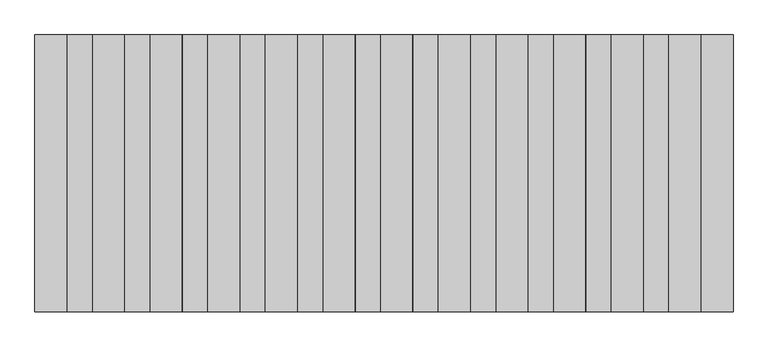
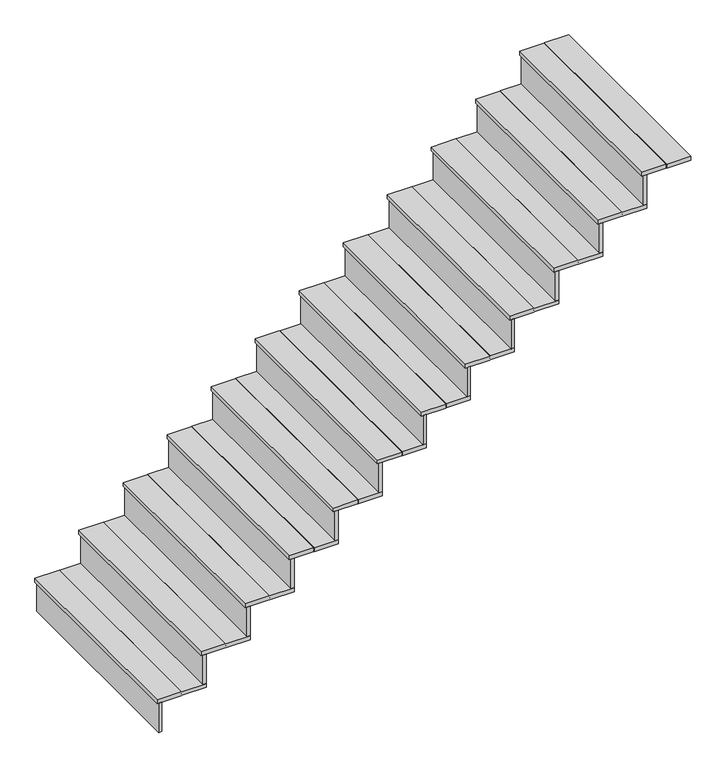
"""IFC4 building model written with IfcOpenShell, lengths in millimetres: stair flight geometry."""

from ifc_helpers import new_model, si_unit, frame, origin, place, context, project, spatial, polyline, outline, extrude, source, transform, mapped, element, save


def stair_flight_ee30e5b9(model_context):
    return source(origin(), model_context, "Body", "SweptSolid", [
        extrude(outline(polyline([(7016.9566393, -79669.5176951), (6997.9066393, -79669.5176951), (6997.9066393, -78450.3176951), (7016.9566393, -78450.3176951), (7016.9566393, -79669.5176951)])), frame((0.0, 0.0, -2438.4), z_axis=(0.0, 0.0, 1.0), x_axis=(1.0, 0.0, 0.0)), (0.0, 0.0, 1.0), 179.2882813),
        extrude(outline(polyline([(-2259.1117187, 7128.0816393), (-2247.3574467, 7128.0816393), (-2247.3574467, 7131.2566393), (-2259.1117188, 7131.2566393), (-2259.1117188, 7270.9566393), (-2235.2, 7270.9566393), (-2235.2, 7131.2566393), (-2246.9542721, 7131.2566393), (-2246.9542721, 7128.0816393), (-2235.2, 7128.0816393), (-2235.2, 6988.3816393), (-2259.1117187, 6988.3816393), (-2259.1117187, 7128.0816393)])), frame((0.0, -79669.5176951, 0.0), z_axis=(0.0, 1.0, 0.0), x_axis=(0.0, 0.0, 1.0)), (0.0, 0.0, 1.0), 1219.2),
        extrude(outline(polyline([(7270.9566393, -79669.5176951), (7251.9066393, -79669.5176951), (7251.9066393, -78450.3176951), (7270.9566393, -78450.3176951), (7270.9566393, -79669.5176951)])), frame((0.0, 0.0, -2235.2), z_axis=(0.0, 0.0, 1.0), x_axis=(1.0, 0.0, 0.0)), (0.0, 0.0, 1.0), 179.2882813),
        extrude(outline(polyline([(-2055.9117188, 7382.0816393), (-2044.1574467, 7382.0816393), (-2044.1574467, 7385.2566393), (-2055.9117188, 7385.2566393), (-2055.9117188, 7524.9566393), (-2032.0, 7524.9566393), (-2032.0, 7385.2566393), (-2043.7542721, 7385.2566393), (-2043.7542721, 7382.0816393), (-2032.0, 7382.0816393), (-2032.0, 7242.3816393), (-2055.9117188, 7242.3816393), (-2055.9117188, 7382.0816393)])), frame((0.0, -79669.5176951, 0.0), z_axis=(0.0, 1.0, 0.0), x_axis=(0.0, 0.0, 1.0)), (0.0, 0.0, 1.0), 1219.2),
        extrude(outline(polyline([(7524.9566393, -79669.5176951), (7505.9066393, -79669.5176951), (7505.9066393, -78450.3176951), (7524.9566393, -78450.3176951), (7524.9566393, -79669.5176951)])), frame((0.0, 0.0, -2032.0), z_axis=(0.0, 0.0, 1.0), x_axis=(1.0, 0.0, 0.0)), (0.0, 0.0, 1.0), 179.2882813),
        extrude(outline(polyline([(-1852.7117188, 7636.0816393), (-1840.9574467, 7636.0816393), (-1840.9574467, 7639.2566393), (-1852.7117188, 7639.2566393), (-1852.7117188, 7778.9566393), (-1828.8, 7778.9566393), (-1828.8, 7639.2566393), (-1840.5542721, 7639.2566393), (-1840.5542721, 7636.0816393), (-1828.8, 7636.0816393), (-1828.8, 7496.3816393), (-1852.7117188, 7496.3816393), (-1852.7117188, 7636.0816393)])), frame((0.0, -79669.5176951, 0.0), z_axis=(0.0, 1.0, 0.0), x_axis=(0.0, 0.0, 1.0)), (0.0, 0.0, 1.0), 1219.2),
        extrude(outline(polyline([(7778.9566393, -79669.5176951), (7759.9066393, -79669.5176951), (7759.9066393, -78450.3176951), (7778.9566393, -78450.3176951), (7778.9566393, -79669.5176951)])), frame((0.0, 0.0, -1828.8), z_axis=(0.0, 0.0, 1.0), x_axis=(1.0, 0.0, 0.0)), (0.0, 0.0, 1.0), 179.2882813),
        extrude(outline(polyline([(-1649.5117188, 7890.0816393), (-1637.7574467, 7890.0816393), (-1637.7574467, 7893.2566393), (-1649.5117188, 7893.2566393), (-1649.5117188, 8032.9566393), (-1625.6, 8032.9566393), (-1625.6, 7893.2566393), (-1637.3542721, 7893.2566393), (-1637.3542721, 7890.0816393), (-1625.6, 7890.0816393), (-1625.6, 7750.3816393), (-1649.5117188, 7750.3816393), (-1649.5117188, 7890.0816393)])), frame((0.0, -79669.5176951, 0.0), z_axis=(0.0, 1.0, 0.0), x_axis=(0.0, 0.0, 1.0)), (0.0, 0.0, 1.0), 1219.2),
        extrude(outline(polyline([(8032.9566393, -79669.5176951), (8013.9066393, -79669.5176951), (8013.9066393, -78450.3176951), (8032.9566393, -78450.3176951), (8032.9566393, -79669.5176951)])), frame((0.0, 0.0, -1625.6), z_axis=(0.0, 0.0, 1.0), x_axis=(1.0, 0.0, 0.0)), (0.0, 0.0, 1.0), 179.2882813),
        extrude(outline(polyline([(-1446.3117187, 8144.0816393), (-1434.5574467, 8144.0816393), (-1434.5574467, 8147.2566393), (-1446.3117188, 8147.2566393), (-1446.3117188, 8286.9566393), (-1422.4, 8286.9566393), (-1422.4, 8147.2566393), (-1434.1542721, 8147.2566393), (-1434.1542721, 8144.0816393), (-1422.4, 8144.0816393), (-1422.4, 8004.3816393), (-1446.3117187, 8004.3816393), (-1446.3117187, 8144.0816393)])), frame((0.0, -79669.5176951, 0.0), z_axis=(0.0, 1.0, 0.0), x_axis=(0.0, 0.0, 1.0)), (0.0, 0.0, 1.0), 1219.2),
        extrude(outline(polyline([(8286.9566393, -79669.5176951), (8267.9066393, -79669.5176951), (8267.9066393, -78450.3176951), (8286.9566393, -78450.3176951), (8286.9566393, -79669.5176951)])), frame((0.0, 0.0, -1422.4), z_axis=(0.0, 0.0, 1.0), x_axis=(1.0, 0.0, 0.0)), (0.0, 0.0, 1.0), 179.2882813),
        extrude(outline(polyline([(-1243.1117187, 8398.0816393), (-1231.3574467, 8398.0816393), (-1231.3574467, 8401.2566393), (-1243.1117188, 8401.2566393), (-1243.1117188, 8540.9566393), (-1219.2, 8540.9566393), (-1219.2, 8401.2566393), (-1230.9542721, 8401.2566393), (-1230.9542721, 8398.0816393), (-1219.2, 8398.0816393), (-1219.2, 8258.3816393), (-1243.1117187, 8258.3816393), (-1243.1117187, 8398.0816393)])), frame((0.0, -79669.5176951, 0.0), z_axis=(0.0, 1.0, 0.0), x_axis=(0.0, 0.0, 1.0)), (0.0, 0.0, 1.0), 1219.2),
        extrude(outline(polyline([(8540.9566393, -79669.5176951), (8521.9066393, -79669.5176951), (8521.9066393, -78450.3176951), (8540.9566393, -78450.3176951), (8540.9566393, -79669.5176951)])), frame((0.0, 0.0, -1219.2), z_axis=(0.0, 0.0, 1.0), x_axis=(1.0, 0.0, 0.0)), (0.0, 0.0, 1.0), 179.2882813),
        extrude(outline(polyline([(-1039.9117188, 8652.0816393), (-1028.1574467, 8652.0816393), (-1028.1574467, 8655.2566393), (-1039.9117188, 8655.2566393), (-1039.9117188, 8794.9566393), (-1016.0, 8794.9566393), (-1016.0, 8655.2566393), (-1027.7542721, 8655.2566393), (-1027.7542721, 8652.0816393), (-1016.0, 8652.0816393), (-1016.0, 8512.3816393), (-1039.9117188, 8512.3816393), (-1039.9117188, 8652.0816393)])), frame((0.0, -79669.5176951, 0.0), z_axis=(0.0, 1.0, 0.0), x_axis=(0.0, 0.0, 1.0)), (0.0, 0.0, 1.0), 1219.2),
        extrude(outline(polyline([(8794.9566393, -79669.5176951), (8775.9066393, -79669.5176951), (8775.9066393, -78450.3176951), (8794.9566393, -78450.3176951), (8794.9566393, -79669.5176951)])), frame((0.0, 0.0, -1016.0), z_axis=(0.0, 0.0, 1.0), x_axis=(1.0, 0.0, 0.0)), (0.0, 0.0, 1.0), 179.2882813),
        extrude(outline(polyline([(-836.7117188, 8906.0816393), (-824.9574467, 8906.0816393), (-824.9574467, 8909.2566393), (-836.7117188, 8909.2566393), (-836.7117188, 9048.9566393), (-812.8, 9048.9566393), (-812.8, 8909.2566393), (-824.5542721, 8909.2566393), (-824.5542721, 8906.0816393), (-812.8, 8906.0816393), (-812.8, 8766.3816393), (-836.7117188, 8766.3816393), (-836.7117188, 8906.0816393)])), frame((0.0, -79669.5176951, 0.0), z_axis=(0.0, 1.0, 0.0), x_axis=(0.0, 0.0, 1.0)), (0.0, 0.0, 1.0), 1219.2),
        extrude(outline(polyline([(9048.9566393, -79669.5176951), (9029.9066393, -79669.5176951), (9029.9066393, -78450.3176951), (9048.9566393, -78450.3176951), (9048.9566393, -79669.5176951)])), frame((0.0, 0.0, -812.8), z_axis=(0.0, 0.0, 1.0), x_axis=(1.0, 0.0, 0.0)), (0.0, 0.0, 1.0), 179.2882813),
        extrude(outline(polyline([(-633.5117188, 9160.0816393), (-621.7574467, 9160.0816393), (-621.7574467, 9163.2566393), (-633.5117188, 9163.2566393), (-633.5117188, 9302.9566393), (-609.6, 9302.9566393), (-609.6, 9163.2566393), (-621.3542721, 9163.2566393), (-621.3542721, 9160.0816393), (-609.6, 9160.0816393), (-609.6, 9020.3816393), (-633.5117188, 9020.3816393), (-633.5117188, 9160.0816393)])), frame((0.0, -79669.5176951, 0.0), z_axis=(0.0, 1.0, 0.0), x_axis=(0.0, 0.0, 1.0)), (0.0, 0.0, 1.0), 1219.2),
        extrude(outline(polyline([(9302.9566393, -79669.5176951), (9283.9066393, -79669.5176951), (9283.9066393, -78450.3176951), (9302.9566393, -78450.3176951), (9302.9566393, -79669.5176951)])), frame((0.0, 0.0, -609.6), z_axis=(0.0, 0.0, 1.0), x_axis=(1.0, 0.0, 0.0)), (0.0, 0.0, 1.0), 179.2882813),
        extrude(outline(polyline([(-430.3117188, 9414.0816393), (-418.5574467, 9414.0816393), (-418.5574467, 9417.2566393), (-430.3117188, 9417.2566393), (-430.3117188, 9556.9566393), (-406.4, 9556.9566393), (-406.4, 9417.2566393), (-418.1542721, 9417.2566393), (-418.1542721, 9414.0816393), (-406.4, 9414.0816393), (-406.4, 9274.3816393), (-430.3117188, 9274.3816393), (-430.3117188, 9414.0816393)])), frame((0.0, -79669.5176951, 0.0), z_axis=(0.0, 1.0, 0.0), x_axis=(0.0, 0.0, 1.0)), (0.0, 0.0, 1.0), 1219.2),
        extrude(outline(polyline([(9556.9566393, -79669.5176951), (9537.9066393, -79669.5176951), (9537.9066393, -78450.3176951), (9556.9566393, -78450.3176951), (9556.9566393, -79669.5176951)])), frame((0.0, 0.0, -406.4), z_axis=(0.0, 0.0, 1.0), x_axis=(1.0, 0.0, 0.0)), (0.0, 0.0, 1.0), 179.2882813),
        extrude(outline(polyline([(-227.1117187, 9668.0816393), (-215.3574467, 9668.0816393), (-215.3574467, 9671.2566393), (-227.1117188, 9671.2566393), (-227.1117188, 9810.9566393), (-203.2, 9810.9566393), (-203.2, 9671.2566393), (-214.9542721, 9671.2566393), (-214.9542721, 9668.0816393), (-203.2, 9668.0816393), (-203.2, 9528.3816393), (-227.1117187, 9528.3816393), (-227.1117187, 9668.0816393)])), frame((0.0, -79669.5176951, 0.0), z_axis=(0.0, 1.0, 0.0), x_axis=(0.0, 0.0, 1.0)), (0.0, 0.0, 1.0), 1219.2),
        extrude(outline(polyline([(9810.9566393, -79669.5176951), (9791.9066393, -79669.5176951), (9791.9066393, -78450.3176951), (9810.9566393, -78450.3176951), (9810.9566393, -79669.5176951)])), frame((0.0, 0.0, -203.2), z_axis=(0.0, 0.0, 1.0), x_axis=(1.0, 0.0, 0.0)), (0.0, 0.0, 1.0), 179.2882812),
        extrude(outline(polyline([(-23.9117188, 9922.0816393), (-12.1574467, 9922.0816393), (-12.1574467, 9925.2566393), (-23.9117188, 9925.2566393), (-23.9117188, 10064.9566393), (0.0, 10064.9566393), (0.0, 9925.2566393), (-11.7542721, 9925.2566393), (-11.7542721, 9922.0816393), (0.0, 9922.0816393), (0.0, 9782.3816393), (-23.9117188, 9782.3816393), (-23.9117188, 9922.0816393)])), frame((0.0, -79669.5176951, 0.0), z_axis=(0.0, 1.0, 0.0), x_axis=(0.0, 0.0, 1.0)), (0.0, 0.0, 1.0), 1219.2),
    ])


if __name__ == "__main__":
    model = new_model("IFC4")
    model_context = context("Model", 3, world=origin())
    ifc_project = project(units=[si_unit("LENGTHUNIT", "METRE", prefix="MILLI")], contexts=[model_context])
    site = spatial("IfcSite", under=ifc_project)
    building = spatial("IfcBuilding", under=site)
    placement = place(None, origin())
    stair_flight_shape = stair_flight_ee30e5b9(model_context)
    element("IfcStairFlight", 1, at=placement, inside=building, context=model_context, shape_type="MappedRepresentation", body=[
        mapped(stair_flight_shape, transform((0.0, 0.0, 0.0), x_axis=(1.0, 0.0, 0.0), y_axis=(0.0, 1.0, 0.0), z_axis=(0.0, 0.0, 1.0))),
    ])
    save(model, "model.ifc")

# Revit data of these elements
# Element 1 (IfcStairFlight)
#   Materials on its faces: "COMPOSITE DECKING"
# Materials
#   "COMPOSITE DECKING": class "Wood", colour RGB 120 75 45, transparency 0, Keynote = "06 11 00", Model = "Trex Select® Composite Deck 1\" Grooved Edge Board", Manufacturer = "Trex", URL = "http://www.trex.com/", Description = "1x6 Trex Select® Composite Deck Grooved Edge Board", Cost = 0
